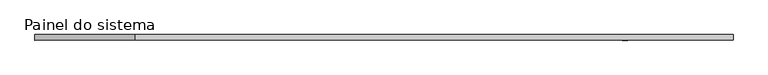
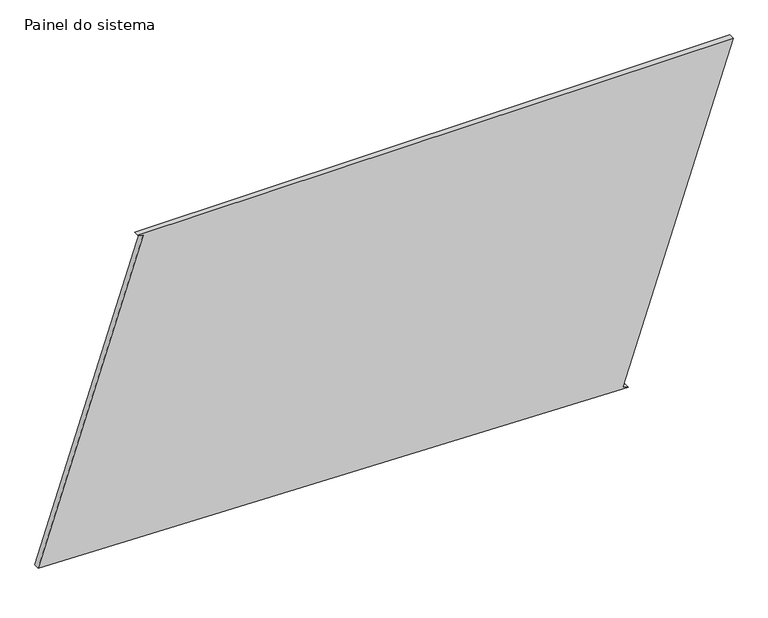
"""IFC4 building model written with IfcOpenShell, lengths in millimetres: plate geometry, Painel do sistema : Envidraçado."""

import ifcopenshell
import ifcopenshell.guid

model = None  # the IFC model being written
_history = None  # IfcOwnerHistory: only IFC2X3 demands one
_inside = {}  # id of a spatial element -> (the spatial element, [elements in it])
_under = {}  # id of a project, library or spatial element -> (it, [spatial elements below it])
_declared = {}  # id of a project -> (the project, [libraries it declares])
_typed = {}  # id of a type object -> (the type object, [elements of that type])
_made_of = {}  # id of a material, layer set ... -> (it, [elements and type objects made of it])


def new_model(schema):
    """Start an empty IFC model of exactly this schema.

    Asked for "IFC4X3", IfcOpenShell would pick the latest addendum, in which some entities
    have other attributes; the version numbers below select the first issue.
    IFC2X3 requires an IfcOwnerHistory on every rooted entity: one is made here for all.
    """
    global model, _history
    if schema == "IFC4X3":
        model = ifcopenshell.file(schema_version=(4, 3, 0, 0))
    else:
        model = ifcopenshell.file(schema=schema)
    _inside.clear()
    _under.clear()
    _declared.clear()
    _typed.clear()
    _made_of.clear()
    _history = None
    if model.schema == "IFC2X3":
        org = make("IfcOrganization", Name="unknown")
        user = make(
            "IfcPersonAndOrganization",
            ThePerson=make("IfcPerson", FamilyName="unknown"),
            TheOrganization=org,
        )
        app = make(
            "IfcApplication",
            ApplicationDeveloper=org,
            Version="unknown",
            ApplicationFullName="unknown",
            ApplicationIdentifier="unknown",
        )
        _history = make(
            "IfcOwnerHistory",
            OwningUser=user,
            OwningApplication=app,
            ChangeAction="ADDED",
            CreationDate=0,
        )
    return model


def make(cls, **values):
    """One entity of the class cls with the attributes given. An attribute that is None is left unset."""
    return model.create_entity(
        cls, **{name: value for name, value in values.items() if value is not None}
    )


def rooted(cls, **values):
    """An entity with a GlobalId (a new one), such as an element, a storey or a relation."""
    return make(cls, GlobalId=ifcopenshell.guid.new(), OwnerHistory=_history, **values)


def si_unit(unit_type, name, prefix=None):
    """IfcSIUnit, for example si_unit("LENGTHUNIT", "METRE", prefix="MILLI")."""
    return make("IfcSIUnit", UnitType=unit_type, Prefix=prefix, Name=name)


def assignment(units):
    """IfcUnitAssignment: the units of a project."""
    return None if units is None else make("IfcUnitAssignment", Units=units)


def point(xyz):
    """IfcCartesianPoint."""
    return None if xyz is None else make("IfcCartesianPoint", Coordinates=xyz)


def direction(xyz):
    """IfcDirection."""
    return None if xyz is None else make("IfcDirection", DirectionRatios=xyz)


def frame(location, z_axis=None, x_axis=None):
    """IfcAxis2Placement3D, a coordinate frame: its origin and axes. An axis left out is left unset."""
    return make(
        "IfcAxis2Placement3D",
        Location=point(location),
        Axis=direction(z_axis),
        RefDirection=direction(x_axis),
    )


def origin():
    """The frame at (0, 0, 0) with its axes left unset."""
    return frame((0.0, 0.0, 0.0))


def place(relative_to, where):
    """IfcLocalPlacement: puts the frame where relative to a parent placement (None: the world)."""
    return make(
        "IfcLocalPlacement", PlacementRelTo=relative_to, RelativePlacement=where
    )


def context(
    kind, dimensions, precision=None, world=None, true_north=None, identifier=None
):
    """IfcGeometricRepresentationContext, for example the 3D "Model" context."""
    return make(
        "IfcGeometricRepresentationContext",
        ContextIdentifier=identifier,
        ContextType=kind,
        CoordinateSpaceDimension=dimensions,
        Precision=precision,
        WorldCoordinateSystem=world,
        TrueNorth=true_north,
    )


def project(units=None, contexts=None):
    """IfcProject with its units and contexts."""
    return rooted(
        "IfcProject",
        Name="project",
        RepresentationContexts=contexts,
        UnitsInContext=assignment(units),
    )


def spatial(cls, under=None, at=None, **own):
    """A site, building, storey or space (cls), placed at a placement, below another one or the project."""
    s = rooted(cls, ObjectPlacement=at, **own)
    if under is not None:
        _under.setdefault(under.id(), (under, []))[1].append(s)
    return s


def polyline(points):
    """IfcPolyline through the points."""
    return make("IfcPolyline", Points=[point(p) for p in points])


def outline(outer, holes=None, kind="AREA"):
    """IfcArbitraryClosedProfileDef: a profile drawn as a closed curve; with holes, ...WithVoids."""
    if holes is None:
        return make("IfcArbitraryClosedProfileDef", ProfileType=kind, OuterCurve=outer)
    return make(
        "IfcArbitraryProfileDefWithVoids",
        ProfileType=kind,
        OuterCurve=outer,
        InnerCurves=holes,
    )


def extrude(swept, where, along, depth):
    """IfcExtrudedAreaSolid: the profile swept, set in the frame where, extruded along a direction by depth."""
    return make(
        "IfcExtrudedAreaSolid",
        SweptArea=swept,
        Position=where,
        ExtrudedDirection=direction(along),
        Depth=depth,
    )


def shape(context_of_items, identifier, shape_type, items):
    """IfcShapeRepresentation: the items that make up one representation, for example the "Body"."""
    return make(
        "IfcShapeRepresentation",
        ContextOfItems=context_of_items,
        RepresentationIdentifier=identifier,
        RepresentationType=shape_type,
        Items=items,
    )


def source(mapping_origin, context_of_items, identifier, shape_type, items):
    """IfcRepresentationMap: a shape defined once, which mapped items show again and again."""
    return make(
        "IfcRepresentationMap",
        MappingOrigin=mapping_origin,
        MappedRepresentation=shape(context_of_items, identifier, shape_type, items),
    )


def transform(
    local_origin,
    x_axis=None,
    y_axis=None,
    z_axis=None,
    scale=None,
    scale2=None,
    scale3=None,
    uniform=True,
):
    """IfcCartesianTransformationOperator3D, or its non-uniform kind. x_axis, y_axis, z_axis: its Axis1, 2, 3."""
    if uniform:
        return make(
            "IfcCartesianTransformationOperator3D",
            Axis1=direction(x_axis),
            Axis2=direction(y_axis),
            LocalOrigin=point(local_origin),
            Scale=scale,
            Axis3=direction(z_axis),
        )
    return make(
        "IfcCartesianTransformationOperator3DnonUniform",
        Axis1=direction(x_axis),
        Axis2=direction(y_axis),
        LocalOrigin=point(local_origin),
        Scale=scale,
        Axis3=direction(z_axis),
        Scale2=scale2,
        Scale3=scale3,
    )


def mapped(mapping_source, mapping_target):
    """IfcMappedItem: shows the shape of a source again, moved by a transform."""
    return make(
        "IfcMappedItem", MappingSource=mapping_source, MappingTarget=mapping_target
    )


def made_of(thing, what):
    """Note that an element or type object is made of a material, layer set ...; save() writes the relation."""
    if what is not None:
        _made_of.setdefault(what.id(), (what, []))[1].append(thing)
    return thing


def element(
    cls,
    number,
    at=None,
    inside=None,
    cuts=None,
    type_object=None,
    material=None,
    context=None,
    identifier="Body",
    shape_type=None,
    held_by="IfcProductDefinitionShape",
    body=None,
    shapes=None,
    **own,
):
    """One element of the class cls, such as IfcWall. Its Tag is "e" and its number.

    at: its placement. inside: the storey or other place that contains it. cuts: it is an
    opening in that element (IfcRelVoidsElement). A single representation is given by context,
    identifier, shape_type and body (its items); several are given by shapes. held_by: the class
    of the entity that holds the representations. save() writes the other relations.
    """
    e = rooted(cls, Tag="e%d" % number, ObjectPlacement=at, **own)
    if body is not None:
        shapes = [shape(context, identifier, shape_type, body)]
    if shapes is not None:
        e.Representation = make(held_by, Representations=shapes)
    if inside is not None:
        _inside.setdefault(inside.id(), (inside, []))[1].append(e)
    if cuts is not None:
        rooted(
            "IfcRelVoidsElement", RelatingBuildingElement=cuts, RelatedOpeningElement=e
        )
    if type_object is not None:
        _typed.setdefault(type_object.id(), (type_object, []))[1].append(e)
    return made_of(e, material)


def aggregate(whole, parts):
    """IfcRelAggregates: a whole, such as a stair, and the parts it consists of."""
    return rooted("IfcRelAggregates", RelatingObject=whole, RelatedObjects=parts)


def save(model, path):
    """Write the relations noted so far, then the file.

    IfcRelAggregates (storeys below a building ...), IfcRelContainedInSpatialStructure (elements
    in a storey), IfcRelDefinesByType, IfcRelAssociatesMaterial and IfcRelDeclares: one each for
    every whole, place, type object, material and project.
    """
    for whole, parts in _under.values():
        aggregate(whole, parts)
    for where, things in _inside.values():
        rooted(
            "IfcRelContainedInSpatialStructure",
            RelatedElements=things,
            RelatingStructure=where,
        )
    for kind, things in _typed.values():
        rooted("IfcRelDefinesByType", RelatedObjects=things, RelatingType=kind)
    for what, things in _made_of.values():
        rooted("IfcRelAssociatesMaterial", RelatedObjects=things, RelatingMaterial=what)
    for by, libraries in _declared.values():
        rooted("IfcRelDeclares", RelatingContext=by, RelatedDefinitions=libraries)
    model.write(path)


def painel_do_sistema_915c0469(model_context):
    return source(origin(), model_context, "Body", "SweptSolid", [
        extrude(outline(polyline([(0.0, 1094.4696143), (7.8961296, 1070.7493458), (1499.7205748, 1567.3558334), (1499.7205748, -1117.72016), (1491.8244452, -1093.9998915), (69.8455081, -1567.3558334), (0.0, 1094.4696143)])), frame((0.0, 24.5, 0.0), z_axis=(0.0, 1.0, 0.0), x_axis=(0.0, 0.0, 1.0)), (0.0, 0.0, 1.0), 25.0),
    ])


if __name__ == "__main__":
    model = new_model("IFC4")
    model_context = context("Model", 3, world=origin())
    ifc_project = project(units=[si_unit("LENGTHUNIT", "METRE", prefix="MILLI")], contexts=[model_context])
    site = spatial("IfcSite", under=ifc_project)
    building = spatial("IfcBuilding", under=site)
    placement = place(None, origin())
    painel_do_sistema_shape = painel_do_sistema_915c0469(model_context)
    element("IfcPlate", 1, ObjectType="Painel do sistema : Envidraçado", at=placement, inside=building, context=model_context, shape_type="MappedRepresentation", body=[
        mapped(painel_do_sistema_shape, transform((0.0, 0.0, 0.0), x_axis=(1.0, 0.0, 0.0), y_axis=(0.0, 1.0, 0.0), z_axis=(0.0, 0.0, 1.0))),
    ])
    save(model, "model.ifc")

# Revit data of these elements
# Type "Painel do sistema : Envidraçado"
#   Construction Type Id = "GSP4R"
#   Analytic Construction = "Vidraça única Pilkington 1/8 pol"
#   Visual Light Transmittance = 0.9
#   Solar Heat Gain Coefficient = 0.86
#   Heat Transfer Coefficient (U) = 6.7069 W/(m²·K)
# Element 1 (IfcPlate, "Painel do sistema : Envidraçado")
#   Materials on its faces: "Vidro"
# Materials
#   "Vidro": class "Vidro", colour RGB 0 128 192, transparency 0.9, Description = "Vidro de sílica", Cost = 0
